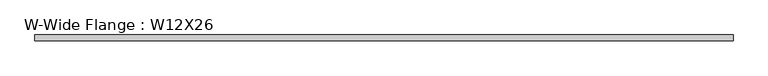
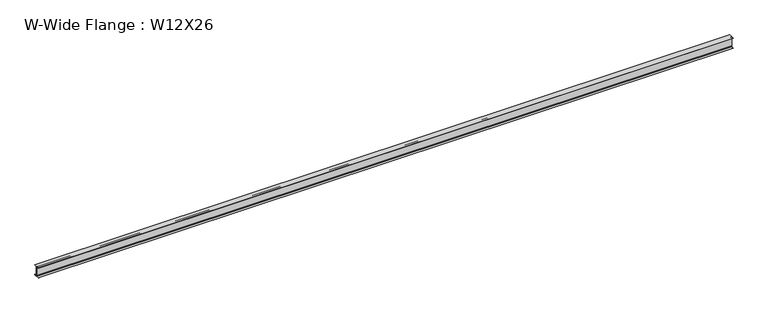
"""IFC4 building model written with IfcOpenShell, lengths in millimetres: beam geometry, W-Wide Flange : W12X26."""

from ifc_helpers import new_model, si_unit, point, frame, frame_2d, origin, place, context, project, spatial, polyline, circle_curve, trimmed, segment, composite_curve, outline, extrude, source, transform, mapped, element, save


def w_wide_flange_w12x26_078f365e(model_context):
    return source(origin(), model_context, "Body", "SweptSolid", [
        extrude(outline(composite_curve([segment(polyline([(82.4011719, -145.5539063), (82.4011719, -155.178125), (-82.4011719, -155.178125), (-82.4011719, -145.5539063), (-20.2902344, -145.5539063)]), True, "CONTINUOUS"), segment(trimmed(circle_curve(frame_2d((-20.2902344, -128.190625)), 17.3632812), [point((-20.2902344, -145.5539063))], [point((-2.9269531, -128.190625))], True, "CARTESIAN"), True, "CONTINUOUS"), segment(polyline([(-2.9269531, -128.190625), (-2.9269531, 128.190625)]), True, "CONTINUOUS"), segment(trimmed(circle_curve(frame_2d((-20.2902344, 128.190625)), 17.3632812), [point((-2.9269531, 128.190625))], [point((-20.2902344, 145.5539062))], True, "CARTESIAN"), True, "CONTINUOUS"), segment(polyline([(-20.2902344, 145.5539062), (-82.4011719, 145.5539062), (-82.4011719, 155.178125), (82.4011719, 155.178125), (82.4011719, 145.5539062), (20.2902344, 145.5539062)]), True, "CONTINUOUS"), segment(trimmed(circle_curve(frame_2d((20.2902344, 128.190625)), 17.3632812), [point((20.2902344, 145.5539062))], [point((2.9269531, 128.190625))], True, "CARTESIAN"), True, "CONTINUOUS"), segment(polyline([(2.9269531, 128.190625), (2.9269531, -128.190625)]), True, "CONTINUOUS"), segment(trimmed(circle_curve(frame_2d((20.2902344, -128.190625)), 17.3632812), [point((2.9269531, -128.190625))], [point((20.2902344, -145.5539063))], True, "CARTESIAN"), True, "CONTINUOUS"), segment(polyline([(20.2902344, -145.5539063), (82.4011719, -145.5539063)]), True, "CONTINUOUS")], self_intersect=False)), frame((-10140.8011719, 0.0, 0.0), z_axis=(1.0, 0.0, 0.0), x_axis=(0.0, 1.0, 0.0)), (0.0, 0.0, 1.0), 20089.6636719),
    ])


if __name__ == "__main__":
    model = new_model("IFC4")
    model_context = context("Model", 3, world=origin())
    ifc_project = project(units=[si_unit("LENGTHUNIT", "METRE", prefix="MILLI")], contexts=[model_context])
    site = spatial("IfcSite", under=ifc_project)
    building = spatial("IfcBuilding", under=site)
    placement = place(None, origin())
    w_wide_flange_w12x26_shape = w_wide_flange_w12x26_078f365e(model_context)
    element("IfcBeam", 1, ObjectType="W-Wide Flange : W12X26", at=placement, inside=building, context=model_context, shape_type="MappedRepresentation", body=[
        mapped(w_wide_flange_w12x26_shape, transform((0.0, 0.0, 0.0), x_axis=(1.0, 0.0, 0.0), y_axis=(0.0, 1.0, 0.0), z_axis=(0.0, 0.0, 1.0))),
    ])
    save(model, "model.ifc")

# Revit data of these elements
# Type "W-Wide Flange : W12X26"
#   Assembly Code = "B10"
#   W = 26
#   Length [instance default] = 5' - 0"
#   bf = 0' - 6 125/256"
#   d = 1' - 0 7/32"
#   k = 0' - 1 1/16"
#   k2 = 0' - 0 175/256"
#   tf = 0' - 0 97/256"
#   tw = 0' - 0 59/256"
#   A = 0.053125 SF
#   Structural Material [instance default] = none
# Element 1 (IfcBeam, "W-Wide Flange : W12X26")
#   Structural Material = Dark metal
#   Materials on its faces: "Dark metal"
# Materials
#   "Dark metal": class "Generic", colour RGB 44 29 29, transparency 0, Cost = 0
